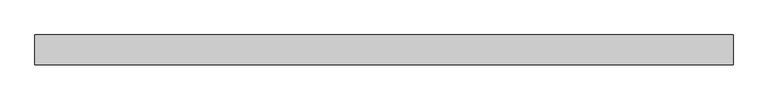
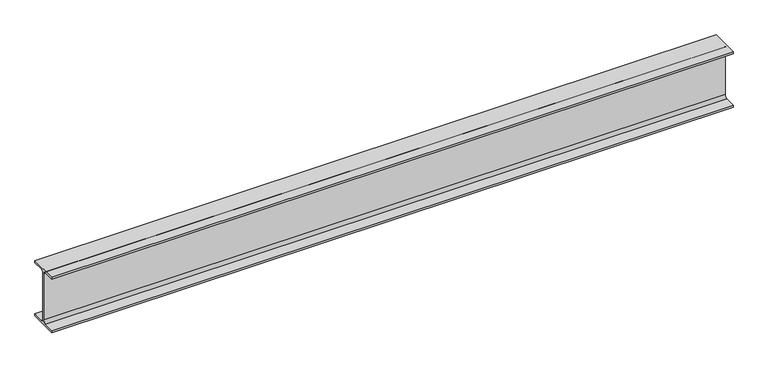
"""IFC4 building model written with IfcOpenShell, lengths in millimetres: beam geometry, 0912_Steel Framing_H-KSD3502 : H_SB_ASB_H-250x125x6x9."""

from ifc_helpers import new_model, si_unit, point, frame, frame_2d, origin, place, context, project, spatial, polyline, circle_curve, trimmed, segment, composite_curve, outline, extrude, source, transform, mapped, element, save


def beam_ed183777(model_context):
    return source(origin(), model_context, "Body", "SweptSolid", [
        extrude(outline(composite_curve([segment(polyline([(62.5, -116.0), (62.5, -125.0), (-62.5, -125.0), (-62.5, -116.0), (-15.0, -116.0)]), True, "CONTINUOUS"), segment(trimmed(circle_curve(frame_2d((-15.0, -104.0)), 12.0), [point((-15.0, -116.0))], [point((-3.0, -104.0))], True, "CARTESIAN"), True, "CONTINUOUS"), segment(polyline([(-3.0, -104.0), (-3.0, 104.0)]), True, "CONTINUOUS"), segment(trimmed(circle_curve(frame_2d((-15.0, 104.0)), 12.0), [point((-3.0, 104.0))], [point((-15.0, 116.0))], True, "CARTESIAN"), True, "CONTINUOUS"), segment(polyline([(-15.0, 116.0), (-62.5, 116.0), (-62.5, 125.0), (62.5, 125.0), (62.5, 116.0), (15.0, 116.0)]), True, "CONTINUOUS"), segment(trimmed(circle_curve(frame_2d((15.0, 104.0)), 12.0), [point((15.0, 116.0))], [point((3.0, 104.0))], True, "CARTESIAN"), True, "CONTINUOUS"), segment(polyline([(3.0, 104.0), (3.0, -104.0)]), True, "CONTINUOUS"), segment(trimmed(circle_curve(frame_2d((15.0, -104.0)), 12.0), [point((3.0, -104.0))], [point((15.0, -116.0))], True, "CARTESIAN"), True, "CONTINUOUS"), segment(polyline([(15.0, -116.0), (62.5, -116.0)]), True, "CONTINUOUS")], self_intersect=False)), frame((-1529.8, 0.0, 0.0), z_axis=(1.0, 0.0, 0.0), x_axis=(0.0, 1.0, 0.0)), (0.0, 0.0, 1.0), 2912.1488581),
    ])


if __name__ == "__main__":
    model = new_model("IFC4")
    model_context = context("Model", 3, world=origin())
    ifc_project = project(units=[si_unit("LENGTHUNIT", "METRE", prefix="MILLI")], contexts=[model_context])
    site = spatial("IfcSite", under=ifc_project)
    building = spatial("IfcBuilding", under=site)
    placement = place(None, origin())
    beam_shape = beam_ed183777(model_context)
    element("IfcBeam", 1, ObjectType="0912_Steel Framing_H-KSD3502 : H_SB_ASB_H-250x125x6x9", at=placement, inside=building, context=model_context, shape_type="MappedRepresentation", body=[
        mapped(beam_shape, transform((0.0, 0.0, 0.0), x_axis=(1.0, 0.0, 0.0), y_axis=(0.0, 1.0, 0.0), z_axis=(0.0, 0.0, 1.0))),
    ])
    save(model, "model.ifc")

# Revit data of these elements
# Type "0912_Steel Framing_H-KSD3502 : H_SB_ASB_H-250x125x6x9"
#   H_WM Code_1 = "S01AA003-00001 | Main Steel Structure Fabrication Work | Shelter/Building | Light Steel - Standard (30KG/M>Weight) | Material: (   )"
#   H_WM Code_2 = "S03AA029-00001 | Main Steel Structure Erection Work | Shelter/Building | Light Steel (30KG/M>Weight) | Material: (   )"
#   H_WM Code_3 = "S01AA010-00001 | Main Steel Structure Fabrication Work | Shelter/Building | Steel Painting/Coating | for Non-Fireproofed Steel Surface, Surface Preparation, Primer, Second & Final Coat | Material: (   )"
#   H_Q'ty Cal Type Tag = "SB-Q2"
#   Width = 12.5 cm
#   Web Thickness = 0.6 cm
#   Web Fillet = 1.2 cm
#   Warping Constant = 42539.8 cm⁶
#   W = 0
#   Torsional Moment of Inertia = 7.8102 cm⁴
#   Section Area = 37.66 cm²
#   Plastic Modulus weak axis = 73.1 cm³
#   Plastic Modulus strong axis = 366.0 cm³
#   Perimeter = 0.97 m²/m
#   Nominal Weight = 29.60 kgf/m
#   Moment of Inertia weak axis = 294.00 cm⁴
#   Moment of Inertia strong axis = 4050.00 cm⁴
#   Height = 25.0 cm
#   Flange Thickness = 0.9 cm
#   Elastic Modulus weak axis = 47.0 cm³
#   Elastic Modulus strong axis = 324.0 cm³
#   Centroid Vertical = 12.5 cm
#   Centroid Horizontal = 6.25 cm
#   Ix = 40500000
#   Length [instance default] = 1.5240 m
#   Zx = 366000
#   b = 0.1250 m
#   h = 0.2500 m
#   r = 0.0120 m
#   s = 0.0060 m
#   t = 0.0090 m
#   A = 0.003766 m²
#   Structural Material [instance default] = Steel, 45-345
#   Assembly Code = ""
# Element 1 (IfcBeam, "0912_Steel Framing_H-KSD3502 : H_SB_ASB_H-250x125x6x9")
#   Structural Material = none
# Materials
#   "Steel, 45-345": class "Metal", colour RGB 189 187 185, transparency 0, Description = "Steel 345 MPa", Cost = 0
